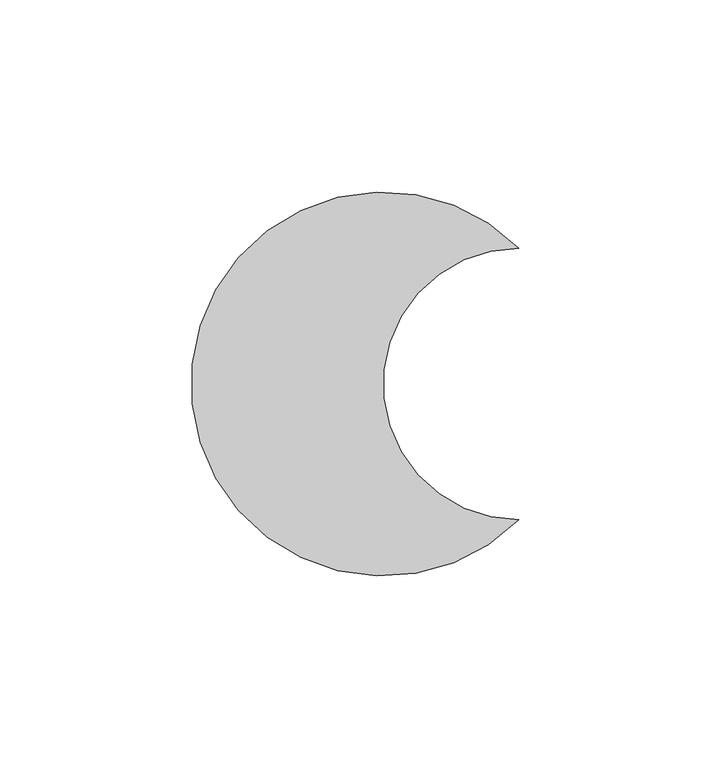
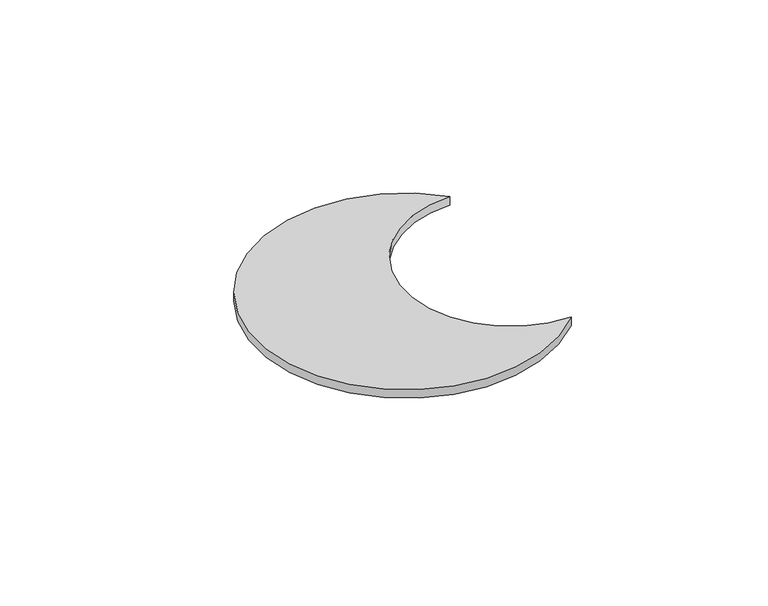
"""IFC4 building model written with IfcOpenShell, lengths in millimetres: proxy geometry, TSPDay and Night Switches : TSPDay and Night Switches."""

from ifc_helpers import new_model, si_unit, point, frame_2d, origin, origin_with_axes, origin_2d, place, context, project, spatial, circle_curve, trimmed, segment, composite_curve, outline, extrude, source, transform, mapped, element, save


def electrical_fixtures_de39ba10(model_context):
    return source(origin(), model_context, "Body", "SweptSolid", [
        extrude(outline(composite_curve([segment(trimmed(circle_curve(origin_2d(), 50.0), [point((35.3553391, -35.3553391))], [point((35.3553391, 35.3553391))], False, "CARTESIAN"), True, "CONTINUOUS"), segment(trimmed(circle_curve(frame_2d((35.3553391, 0.0)), 35.3553391), [point((35.3553391, 35.3553391))], [point((35.3553391, -35.3553391))], True, "CARTESIAN"), True, "CONTINUOUS")], self_intersect=False)), origin_with_axes(), (0.0, 0.0, 1.0), 3.0),
    ])


if __name__ == "__main__":
    model = new_model("IFC4")
    model_context = context("Model", 3, world=origin())
    ifc_project = project(units=[si_unit("LENGTHUNIT", "METRE", prefix="MILLI")], contexts=[model_context])
    site = spatial("IfcSite", under=ifc_project)
    building = spatial("IfcBuilding", under=site)
    placement = place(None, origin())
    electrical_fixtures_shape = electrical_fixtures_de39ba10(model_context)
    element("IfcBuildingElementProxy", 1, Name="TSPDay and Night Switches : TSPDay and Night Switches", ObjectType="TSPDay and Night Switches : TSPDay and Night Switches", at=placement, inside=building, context=model_context, shape_type="MappedRepresentation", body=[
        mapped(electrical_fixtures_shape, transform((0.0, 0.0, 0.0), x_axis=(1.0, 0.0, 0.0), y_axis=(0.0, 1.0, 0.0), z_axis=(0.0, 0.0, 1.0))),
    ])
    save(model, "model.ifc")

# Revit data of these elements
# Type "TSPDay and Night Switches : TSPDay and Night Switches"
#   Model = "TSP_ELECDNS"
#   Default Elevation = 0
# Element 1 (IfcBuildingElementProxy, "TSPDay and Night Switches : TSPDay and Night Switches")
#   Materials on its faces: "Plastic, Opaque Black"
# Materials
#   "Plastic, Opaque Black": class "Plastic", colour RGB 0 0 0, transparency 0.7, Description = "Plastic, generic, opaque black", Cost = 0
